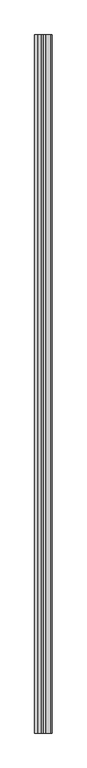
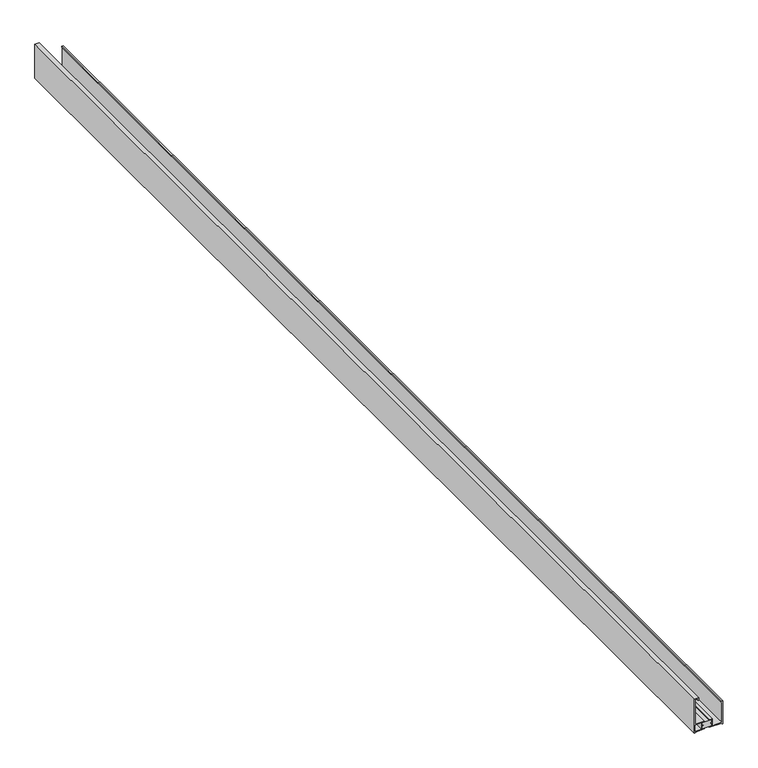
"""IFC4 building model written with IfcOpenShell, lengths in millimetres: proxy geometry, Generic Models 3:Generic Models 2:312240:Generic Models 2:312240 : Generic Models 3:Generic Models 2:312240:4 : Generic Models 3:Generic Models 2:312240:Generic Models 2:312240 : Generic Models 3:Generic Models 2:312240:300533."""

from ifc_helpers import new_model, si_unit, frame, origin, place, context, project, spatial, polyline, outline, extrude, source, transform, mapped, element, save


def generic_models_d5fd764a(model_context):
    return source(origin(), model_context, "Body", "SweptSolid", [
        extrude(outline(polyline([(21.6981223, 667560.2558518), (21.6981223, 667543.7035956), (17.0006236, 667543.7035956), (17.0006236, 667545.6290111), (14.6193736, 667545.6290111), (14.6193736, 667543.7035956), (9.921875, 667543.7035956), (9.921875, 667560.2558518), (14.6193736, 667560.2558518), (14.6193736, 667558.3304364), (17.0006236, 667558.3304364), (17.0006236, 667560.2558518), (21.6981223, 667560.2558518)])), frame((0.0, -503999.8915363, 0.0), z_axis=(0.0, 1.0, 0.0), x_axis=(0.0, 0.0, 1.0)), (0.0, 0.0, 1.0), 2178.6876522),
        extrude(outline(polyline([(74.35, 667536.6662072), (74.35, 667528.2198356), (6.35, 667528.2198356), (6.35, 667529.8073356), (7.9375, 667529.8073356), (7.9375, 667547.4739081), (9.525, 667547.4739081), (9.525, 667543.3067206), (15.0162486, 667543.3067206), (15.0162486, 667545.2321361), (16.6037486, 667545.2321361), (16.6037486, 667543.3067206), (22.0949973, 667543.3067206), (22.0949973, 667547.4739081), (23.6824973, 667547.4739081), (23.6824973, 667529.8073356), (72.7625, 667529.8073356), (72.7625, 667535.0787072), (69.9626734, 667535.0787072), (69.9626734, 667536.6662072), (74.35, 667536.6662072)]), holes=[polyline([(22.0949973, 667529.8073356), (22.0949973, 667541.7192206), (9.525, 667541.7192206), (9.525, 667529.8073356), (22.0949973, 667529.8073356)])]), frame((0.0, -503999.8915363, 0.0), z_axis=(0.0, 1.0, 0.0), x_axis=(0.0, 0.0, 1.0)), (0.0, 0.0, 1.0), 2178.6876522),
        extrude(outline(polyline([(6.35, 667580.6323356), (6.35, 667582.2198356), (52.3546875, 667582.2198356), (52.3546875, 667579.5047457), (50.7671875, 667579.5047457), (50.7671875, 667580.6323356), (9.525, 667580.6323356), (9.525, 667562.2402268), (23.6824973, 667562.2402268), (23.6824973, 667556.4855393), (22.0949973, 667556.4855393), (22.0949973, 667560.6527268), (16.6037486, 667560.6527268), (16.6037486, 667558.7273114), (15.0162486, 667558.7273114), (15.0162486, 667560.6527268), (9.525, 667560.6527268), (9.525, 667556.4855393), (7.9375, 667556.4855393), (7.9375, 667580.6323356), (6.35, 667580.6323356)])), frame((0.0, -503999.8915363, 0.0), z_axis=(0.0, 1.0, 0.0), x_axis=(0.0, 0.0, 1.0)), (0.0, 0.0, 1.0), 2178.6876522),
    ])


if __name__ == "__main__":
    model = new_model("IFC4")
    model_context = context("Model", 3, world=origin())
    ifc_project = project(units=[si_unit("LENGTHUNIT", "METRE", prefix="MILLI")], contexts=[model_context])
    site = spatial("IfcSite", under=ifc_project)
    building = spatial("IfcBuilding", under=site)
    placement = place(None, origin())
    generic_models_shape = generic_models_d5fd764a(model_context)
    element("IfcBuildingElementProxy", 1, Name="Generic Models 3:Generic Models 2:312240:Generic Models 2:312240 : Generic Models 3:Generic Models 2:312240:4 : Generic Models 3:Generic Models 2:312240:Generic Models 2:312240 : Generic Models 3:Generic Models 2:312240:300533", ObjectType="Generic Models 3:Generic Models 2:312240:Generic Models 2:312240 : Generic Models 3:Generic Models 2:312240:4 : Generic Models 3:Generic Models 2:312240:Generic Models 2:312240 : Generic Models 3:Generic Models 2:312240:300533", at=placement, inside=building, context=model_context, shape_type="MappedRepresentation", body=[
        mapped(generic_models_shape, transform((0.0, 0.0, 0.0), x_axis=(1.0, 0.0, 0.0), y_axis=(0.0, 1.0, 0.0), z_axis=(0.0, 0.0, 1.0))),
    ])
    save(model, "model.ifc")

# Revit data of these elements
# Type "Generic Models 3:Generic Models 2:312240:Generic Models 2:312240 : Generic Models 3:Generic Models 2:312240:4 : Generic Models 3:Generic Models 2:312240:Generic Models 2:312240 : Generic Models 3:Generic Models 2:312240:300533"
#   NameOverride = "Generic Models 3:Generic Models 2:312240:Generic Models 2:312240 : Generic Models 3:Generic Models 2:312240:300533"
#   ObjectTypeOverride = "Generic Models 2:312240 : Generic Models 3:Generic Models 2:312240"
#   Reference = "Generic Models 2"
#   Tag = "300533"
# Element 1 (IfcBuildingElementProxy, "Generic Models 3:Generic Models 2:312240:Generic Models 2:312240 : Generic Models 3:Generic Models 2:312240:4 : Generic Models 3:Generic Models 2:312240:Generic Models 2:312240 : Generic Models 3:Generic Models 2:312240:300533")
#   Materials on its faces: "THERMAL BROKEN ALUMINUM STOREFRONT FOR POLYCARBONATE"
# Materials
#   "THERMAL BROKEN ALUMINUM STOREFRONT FOR POLYCARBONATE": class "Unassigned", colour RGB 244 244 244, transparency 0, Keynote = "M07611300.01", Cost = 0
